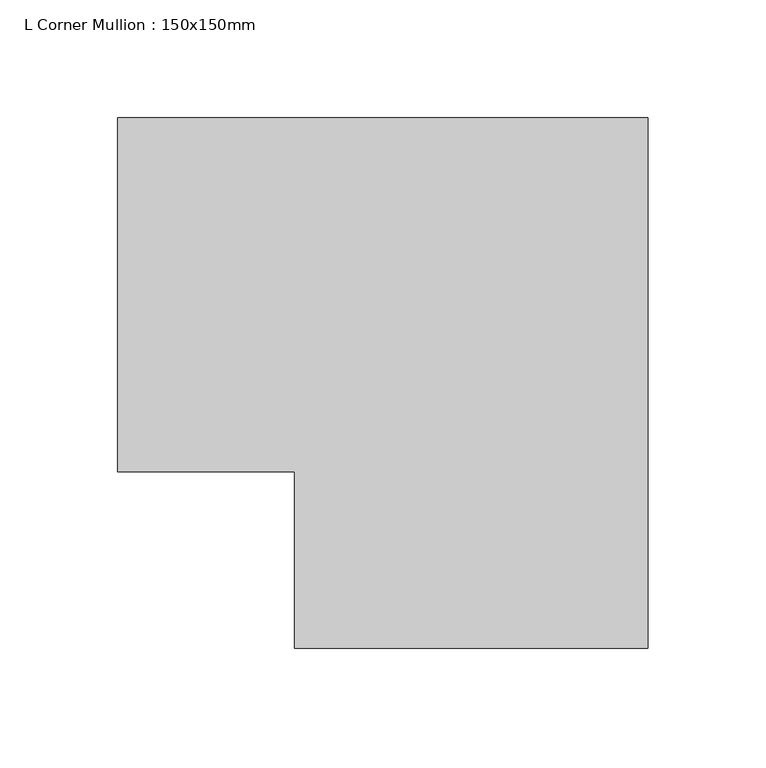
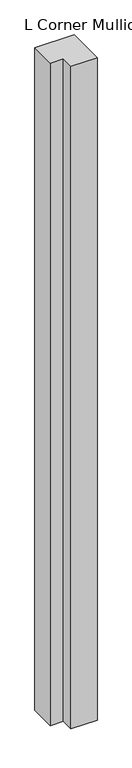
"""IFC4 building model written with IfcOpenShell, lengths in millimetres: member geometry, L Corner Mullion : 150x150mm."""

from ifc_helpers import new_model, si_unit, frame, origin, place, context, project, spatial, polyline, outline, extrude, source, transform, mapped, element, save


def l_corner_mullion_150x150mm_b70191eb(model_context):
    return source(origin(), model_context, "Body", "SweptSolid", [
        extrude(outline(polyline([(-75.0, -150.0), (-75.0, -75.0), (-150.0, -75.0), (-150.0, 75.0), (75.0, 75.0), (75.0, -150.0), (-75.0, -150.0)])), frame((0.0, 0.0, -4000.0), z_axis=(0.0, 0.0, 1.0), x_axis=(1.0, 0.0, 0.0)), (0.0, 0.0, 1.0), 4000.0),
    ])


if __name__ == "__main__":
    model = new_model("IFC4")
    model_context = context("Model", 3, world=origin())
    ifc_project = project(units=[si_unit("LENGTHUNIT", "METRE", prefix="MILLI")], contexts=[model_context])
    site = spatial("IfcSite", under=ifc_project)
    building = spatial("IfcBuilding", under=site)
    placement = place(None, origin())
    l_corner_mullion_150x150mm_shape = l_corner_mullion_150x150mm_b70191eb(model_context)
    element("IfcMember", 1, ObjectType="L Corner Mullion : 150x150mm", at=placement, inside=building, context=model_context, shape_type="MappedRepresentation", body=[
        mapped(l_corner_mullion_150x150mm_shape, transform((0.0, 0.0, 0.0), x_axis=(1.0, 0.0, 0.0), y_axis=(0.0, 1.0, 0.0), z_axis=(0.0, 0.0, 1.0))),
    ])
    save(model, "model.ifc")

# Revit data of these elements
# Type "L Corner Mullion : 150x150mm"
#   Keynote = "H11"
#   built-in parameter 1007355 = 0.492126 (stored number, unit not read)
#   built-in parameter 1007354 = 0.492126 (stored number, unit not read)
#   built-in parameter 1007304 = 0.492126 (stored number, unit not read)
# Element 1 (IfcMember, "L Corner Mullion : 150x150mm")
#   Materials on its faces: "Aluminium"
# Materials
#   "Aluminium": class "Metal", colour RGB 247 247 247, transparency 0, Description = "Aluminium 6061", Cost = 0
